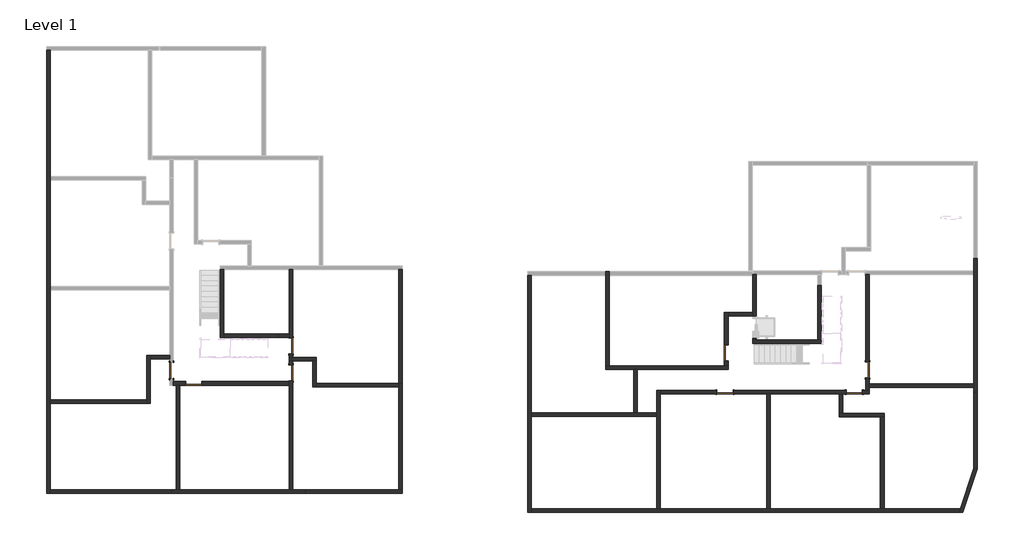
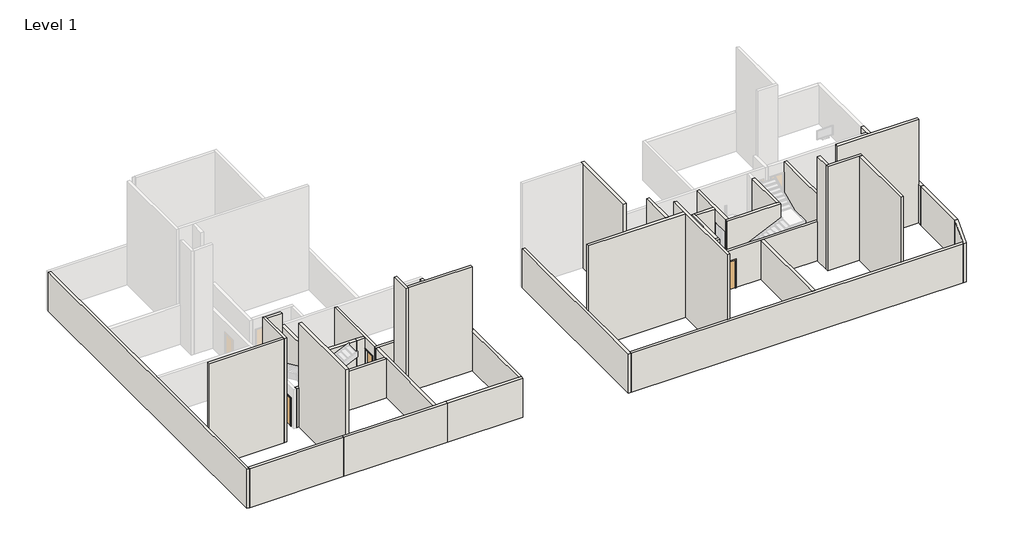
# One storey, part 1 of 2: 41 walls, 8 doors.
"""IFC4 building model written with IfcOpenShell, lengths in millimetres."""

import ifcopenshell
import ifcopenshell.guid

model = None  # the IFC model being written
_history = None  # IfcOwnerHistory: only IFC2X3 demands one
_inside = {}  # id of a spatial element -> (the spatial element, [elements in it])
_under = {}  # id of a project, library or spatial element -> (it, [spatial elements below it])
_declared = {}  # id of a project -> (the project, [libraries it declares])
_typed = {}  # id of a type object -> (the type object, [elements of that type])
_made_of = {}  # id of a material, layer set ... -> (it, [elements and type objects made of it])


def new_model(schema):
    """Start an empty IFC model of exactly this schema.

    Asked for "IFC4X3", IfcOpenShell would pick the latest addendum, in which some entities
    have other attributes; the version numbers below select the first issue.
    IFC2X3 requires an IfcOwnerHistory on every rooted entity: one is made here for all.
    """
    global model, _history
    if schema == "IFC4X3":
        model = ifcopenshell.file(schema_version=(4, 3, 0, 0))
    else:
        model = ifcopenshell.file(schema=schema)
    _inside.clear()
    _under.clear()
    _declared.clear()
    _typed.clear()
    _made_of.clear()
    _history = None
    if model.schema == "IFC2X3":
        org = make("IfcOrganization", Name="unknown")
        user = make(
            "IfcPersonAndOrganization",
            ThePerson=make("IfcPerson", FamilyName="unknown"),
            TheOrganization=org,
        )
        app = make(
            "IfcApplication",
            ApplicationDeveloper=org,
            Version="unknown",
            ApplicationFullName="unknown",
            ApplicationIdentifier="unknown",
        )
        _history = make(
            "IfcOwnerHistory",
            OwningUser=user,
            OwningApplication=app,
            ChangeAction="ADDED",
            CreationDate=0,
        )
    return model


def make(cls, **values):
    """One entity of the class cls with the attributes given. An attribute that is None is left unset."""
    return model.create_entity(
        cls, **{name: value for name, value in values.items() if value is not None}
    )


def rooted(cls, **values):
    """An entity with a GlobalId (a new one), such as an element, a storey or a relation."""
    return make(cls, GlobalId=ifcopenshell.guid.new(), OwnerHistory=_history, **values)


def si_unit(unit_type, name, prefix=None):
    """IfcSIUnit, for example si_unit("LENGTHUNIT", "METRE", prefix="MILLI")."""
    return make("IfcSIUnit", UnitType=unit_type, Prefix=prefix, Name=name)


def assignment(units):
    """IfcUnitAssignment: the units of a project."""
    return None if units is None else make("IfcUnitAssignment", Units=units)


def point(xyz):
    """IfcCartesianPoint."""
    return None if xyz is None else make("IfcCartesianPoint", Coordinates=xyz)


def direction(xyz):
    """IfcDirection."""
    return None if xyz is None else make("IfcDirection", DirectionRatios=xyz)


def frame(location, z_axis=None, x_axis=None):
    """IfcAxis2Placement3D, a coordinate frame: its origin and axes. An axis left out is left unset."""
    return make(
        "IfcAxis2Placement3D",
        Location=point(location),
        Axis=direction(z_axis),
        RefDirection=direction(x_axis),
    )


def origin():
    """The frame at (0, 0, 0) with its axes left unset."""
    return frame((0.0, 0.0, 0.0))


def origin_with_axes():
    """The frame at (0, 0, 0) with the z axis (0, 0, 1) and the x axis (1, 0, 0) written out."""
    return frame((0.0, 0.0, 0.0), z_axis=(0.0, 0.0, 1.0), x_axis=(1.0, 0.0, 0.0))


def place(relative_to, where):
    """IfcLocalPlacement: puts the frame where relative to a parent placement (None: the world)."""
    return make(
        "IfcLocalPlacement", PlacementRelTo=relative_to, RelativePlacement=where
    )


def context(
    kind, dimensions, precision=None, world=None, true_north=None, identifier=None
):
    """IfcGeometricRepresentationContext, for example the 3D "Model" context."""
    return make(
        "IfcGeometricRepresentationContext",
        ContextIdentifier=identifier,
        ContextType=kind,
        CoordinateSpaceDimension=dimensions,
        Precision=precision,
        WorldCoordinateSystem=world,
        TrueNorth=true_north,
    )


def project(units=None, contexts=None):
    """IfcProject with its units and contexts."""
    return rooted(
        "IfcProject",
        Name="project",
        RepresentationContexts=contexts,
        UnitsInContext=assignment(units),
    )


def spatial(cls, under=None, at=None, **own):
    """A site, building, storey or space (cls), placed at a placement, below another one or the project."""
    s = rooted(cls, ObjectPlacement=at, **own)
    if under is not None:
        _under.setdefault(under.id(), (under, []))[1].append(s)
    return s


def polyline(points):
    """IfcPolyline through the points."""
    return make("IfcPolyline", Points=[point(p) for p in points])


def outline(outer, holes=None, kind="AREA"):
    """IfcArbitraryClosedProfileDef: a profile drawn as a closed curve; with holes, ...WithVoids."""
    if holes is None:
        return make("IfcArbitraryClosedProfileDef", ProfileType=kind, OuterCurve=outer)
    return make(
        "IfcArbitraryProfileDefWithVoids",
        ProfileType=kind,
        OuterCurve=outer,
        InnerCurves=holes,
    )


def extrude(swept, where, along, depth):
    """IfcExtrudedAreaSolid: the profile swept, set in the frame where, extruded along a direction by depth."""
    return make(
        "IfcExtrudedAreaSolid",
        SweptArea=swept,
        Position=where,
        ExtrudedDirection=direction(along),
        Depth=depth,
    )


def faces_of(points, faces, orient=None, outer=None):
    """IfcFace entities. A face is a list of loops; a loop is a list of indices into points, from 0.

    orient and outer hold one flag for each loop. By default every Orientation is true, the
    first loop of a face is its IfcFaceOuterBound and the others are IfcFaceBound.
    """
    made = []
    for i, loops in enumerate(faces):
        bounds = []
        for j, loop in enumerate(loops):
            is_outer = j == 0 if outer is None else outer[i][j]
            bounds.append(
                make(
                    "IfcFaceOuterBound" if is_outer else "IfcFaceBound",
                    Bound=make("IfcPolyLoop", Polygon=[points[k] for k in loop]),
                    Orientation=True if orient is None else orient[i][j],
                )
            )
        made.append(make("IfcFace", Bounds=bounds))
    return made


def faceted_brep(points, faces, orient=None, outer=None, voids=None):
    """IfcFacetedBrep: a solid bounded by flat faces; with voids (closed shells), ...WithVoids."""
    shared = [point(p) for p in points]
    hull = make("IfcClosedShell", CfsFaces=faces_of(shared, faces, orient, outer))
    if voids is None:
        return make("IfcFacetedBrep", Outer=hull)
    return make(
        "IfcFacetedBrepWithVoids",
        Outer=hull,
        Voids=[
            make(cls, CfsFaces=faces_of(shared, fs, o, b)) for cls, fs, o, b in voids
        ],
    )


def shape(context_of_items, identifier, shape_type, items):
    """IfcShapeRepresentation: the items that make up one representation, for example the "Body"."""
    return make(
        "IfcShapeRepresentation",
        ContextOfItems=context_of_items,
        RepresentationIdentifier=identifier,
        RepresentationType=shape_type,
        Items=items,
    )


def source(mapping_origin, context_of_items, identifier, shape_type, items):
    """IfcRepresentationMap: a shape defined once, which mapped items show again and again."""
    return make(
        "IfcRepresentationMap",
        MappingOrigin=mapping_origin,
        MappedRepresentation=shape(context_of_items, identifier, shape_type, items),
    )


def transform(
    local_origin,
    x_axis=None,
    y_axis=None,
    z_axis=None,
    scale=None,
    scale2=None,
    scale3=None,
    uniform=True,
):
    """IfcCartesianTransformationOperator3D, or its non-uniform kind. x_axis, y_axis, z_axis: its Axis1, 2, 3."""
    if uniform:
        return make(
            "IfcCartesianTransformationOperator3D",
            Axis1=direction(x_axis),
            Axis2=direction(y_axis),
            LocalOrigin=point(local_origin),
            Scale=scale,
            Axis3=direction(z_axis),
        )
    return make(
        "IfcCartesianTransformationOperator3DnonUniform",
        Axis1=direction(x_axis),
        Axis2=direction(y_axis),
        LocalOrigin=point(local_origin),
        Scale=scale,
        Axis3=direction(z_axis),
        Scale2=scale2,
        Scale3=scale3,
    )


def mapped(mapping_source, mapping_target):
    """IfcMappedItem: shows the shape of a source again, moved by a transform."""
    return make(
        "IfcMappedItem", MappingSource=mapping_source, MappingTarget=mapping_target
    )


def made_of(thing, what):
    """Note that an element or type object is made of a material, layer set ...; save() writes the relation."""
    if what is not None:
        _made_of.setdefault(what.id(), (what, []))[1].append(thing)
    return thing


def element(
    cls,
    number,
    at=None,
    inside=None,
    cuts=None,
    type_object=None,
    material=None,
    context=None,
    identifier="Body",
    shape_type=None,
    held_by="IfcProductDefinitionShape",
    body=None,
    shapes=None,
    **own,
):
    """One element of the class cls, such as IfcWall. Its Tag is "e" and its number.

    at: its placement. inside: the storey or other place that contains it. cuts: it is an
    opening in that element (IfcRelVoidsElement). A single representation is given by context,
    identifier, shape_type and body (its items); several are given by shapes. held_by: the class
    of the entity that holds the representations. save() writes the other relations.
    """
    e = rooted(cls, Tag="e%d" % number, ObjectPlacement=at, **own)
    if body is not None:
        shapes = [shape(context, identifier, shape_type, body)]
    if shapes is not None:
        e.Representation = make(held_by, Representations=shapes)
    if inside is not None:
        _inside.setdefault(inside.id(), (inside, []))[1].append(e)
    if cuts is not None:
        rooted(
            "IfcRelVoidsElement", RelatingBuildingElement=cuts, RelatedOpeningElement=e
        )
    if type_object is not None:
        _typed.setdefault(type_object.id(), (type_object, []))[1].append(e)
    return made_of(e, material)


def aggregate(whole, parts):
    """IfcRelAggregates: a whole, such as a stair, and the parts it consists of."""
    return rooted("IfcRelAggregates", RelatingObject=whole, RelatedObjects=parts)


def save(model, path):
    """Write the relations noted so far, then the file.

    IfcRelAggregates (storeys below a building ...), IfcRelContainedInSpatialStructure (elements
    in a storey), IfcRelDefinesByType, IfcRelAssociatesMaterial and IfcRelDeclares: one each for
    every whole, place, type object, material and project.
    """
    for whole, parts in _under.values():
        aggregate(whole, parts)
    for where, things in _inside.values():
        rooted(
            "IfcRelContainedInSpatialStructure",
            RelatedElements=things,
            RelatingStructure=where,
        )
    for kind, things in _typed.values():
        rooted("IfcRelDefinesByType", RelatedObjects=things, RelatingType=kind)
    for what, things in _made_of.values():
        rooted("IfcRelAssociatesMaterial", RelatedObjects=things, RelatingMaterial=what)
    for by, libraries in _declared.values():
        rooted("IfcRelDeclares", RelatingContext=by, RelatedDefinitions=libraries)
    model.write(path)


def m_single_flush_0915_x_2134mm_727434cd(model_context):
    return source(origin(), model_context, "Body", "SweptSolid", [
        extrude(outline(polyline([(2210.0, -533.5), (0.0, -533.5), (0.0, -457.5), (2134.0, -457.5), (2134.0, 457.5), (0.0, 457.5), (0.0, 533.5), (2210.0, 533.5), (2210.0, -533.5)])), frame((0.0, -125.0, 0.0), z_axis=(0.0, 1.0, 0.0), x_axis=(0.0, 0.0, 1.0)), (0.0, 0.0, 1.0), 25.0),
        extrude(outline(polyline([(2210.0, 533.5), (2210.0, -533.5), (0.0, -533.5), (0.0, -457.5), (2134.0, -457.5), (2134.0, 457.5), (0.0, 457.5), (0.0, 533.5), (2210.0, 533.5)])), frame((0.0, 100.0, 0.0), z_axis=(0.0, 1.0, 0.0), x_axis=(0.0, 0.0, 1.0)), (0.0, 0.0, 1.0), 25.0),
        extrude(outline(polyline([(457.5, -49.0), (457.5, -100.0), (-457.5, -100.0), (-457.5, -49.0), (457.5, -49.0)])), origin_with_axes(), (0.0, 0.0, 1.0), 2134.0),
    ])


def m_single_flush_0915_x_2134mm_6a9e8738(model_context):
    return source(origin(), model_context, "Body", "SweptSolid", [
        extrude(outline(polyline([(2210.0, -533.5), (0.0, -533.5), (0.0, -457.5), (2134.0, -457.5), (2134.0, 457.5), (0.0, 457.5), (0.0, 533.5), (2210.0, 533.5), (2210.0, -533.5)])), frame((0.0, 100.0, 0.0), z_axis=(0.0, 1.0, 0.0), x_axis=(0.0, 0.0, 1.0)), (0.0, 0.0, 1.0), 25.0),
        extrude(outline(polyline([(2210.0, 533.5), (2210.0, -533.5), (0.0, -533.5), (0.0, -457.5), (2134.0, -457.5), (2134.0, 457.5), (0.0, 457.5), (0.0, 533.5), (2210.0, 533.5)])), frame((0.0, -125.0, 0.0), z_axis=(0.0, 1.0, 0.0), x_axis=(0.0, 0.0, 1.0)), (0.0, 0.0, 1.0), 25.0),
        extrude(outline(polyline([(457.5, 49.0), (-457.5, 49.0), (-457.5, 100.0), (457.5, 100.0), (457.5, 49.0)])), origin_with_axes(), (0.0, 0.0, 1.0), 2134.0),
    ])


model = new_model("IFC4")

# Units and contexts
model_context = context("Model", 3, world=origin())
ifc_project = project(units=[si_unit("LENGTHUNIT", "METRE", prefix="MILLI")], contexts=[model_context])

# Site, building, storey
site = spatial("IfcSite", under=ifc_project)
building = spatial("IfcBuilding", under=site)
storey = spatial("IfcBuildingStorey", under=building, Name="Level 1", Elevation=0.0)

# Doors
placement = place(None, origin())
m_single_flush_0915_x_2134mm_shape = m_single_flush_0915_x_2134mm_727434cd(model_context)
element("IfcDoor", 1, ObjectType="M_Single-Flush : 0915 x 2134mm", at=placement, inside=storey, context=model_context, shape_type="MappedRepresentation", body=[
    mapped(m_single_flush_0915_x_2134mm_shape, transform((16070.6041014, -3023.024372, 0.0), x_axis=(0.0, -1.0, 0.0), y_axis=(1.0, 0.0, 0.0), z_axis=(0.0, 0.0, 1.0))),
])
element("IfcDoor", 2, ObjectType="M_Single-Flush : 0915 x 2134mm", at=placement, inside=storey, context=model_context, shape_type="MappedRepresentation", body=[
    mapped(m_single_flush_0915_x_2134mm_shape, transform((16002.336337, -5240.0098119, 0.0), x_axis=(1.0, 0.0, 0.0), y_axis=(0.0, 1.0, 0.0), z_axis=(0.0, 0.0, 1.0))),
])
element("IfcDoor", 3, ObjectType="M_Single-Flush : 0915 x 2134mm", at=placement, inside=storey, context=model_context, shape_type="MappedRepresentation", body=[
    mapped(m_single_flush_0915_x_2134mm_shape, transform((-8530.3449834, -4137.6378151, 0.0), x_axis=(0.0, 1.0, 0.0), y_axis=(-1.0, 0.0, 0.0), z_axis=(0.0, 0.0, 1.0))),
])
m_single_flush_0915_x_2134mm_2_shape = m_single_flush_0915_x_2134mm_6a9e8738(model_context)
element("IfcDoor", 4, ObjectType="M_Single-Flush : 0915 x 2134mm", at=placement, inside=storey, context=model_context, shape_type="MappedRepresentation", body=[
    mapped(m_single_flush_0915_x_2134mm_2_shape, transform((24048.8612349, -3982.5098119, 0.0), x_axis=(0.0, -1.0, 0.0), y_axis=(1.0, 0.0, 0.0), z_axis=(0.0, 0.0, 1.0))),
])
element("IfcDoor", 5, ObjectType="M_Single-Flush : 0915 x 2134mm", at=placement, inside=storey, context=model_context, shape_type="MappedRepresentation", body=[
    mapped(m_single_flush_0915_x_2134mm_2_shape, transform((23308.8612349, -5240.0098119, 0.0), x_axis=(-1.0, 0.0, 0.0), y_axis=(0.0, -1.0, 0.0), z_axis=(0.0, 0.0, 1.0))),
])
element("IfcDoor", 6, ObjectType="M_Single-Flush : 0915 x 2134mm", at=placement, inside=storey, context=model_context, shape_type="MappedRepresentation", body=[
    mapped(m_single_flush_0915_x_2134mm_2_shape, transform((-14032.3304233, -4739.1627129, 0.0), x_axis=(-1.0, 0.0, 0.0), y_axis=(0.0, -1.0, 0.0), z_axis=(0.0, 0.0, 1.0))),
])
element("IfcDoor", 7, ObjectType="M_Single-Flush : 0915 x 2134mm", at=placement, inside=storey, context=model_context, shape_type="MappedRepresentation", body=[
    mapped(m_single_flush_0915_x_2134mm_2_shape, transform((-8530.3449834, -2622.6378151, 0.0), x_axis=(0.0, -1.0, 0.0), y_axis=(1.0, 0.0, 0.0), z_axis=(0.0, 0.0, 1.0))),
])
element("IfcDoor", 8, ObjectType="M_Single-Flush : 0915 x 2134mm", at=placement, inside=storey, context=model_context, shape_type="MappedRepresentation", body=[
    mapped(m_single_flush_0915_x_2134mm_2_shape, transform((-15289.8304233, -3999.1627129, 0.0), x_axis=(0.0, 1.0, 0.0), y_axis=(-1.0, 0.0, 0.0), z_axis=(0.0, 0.0, 1.0))),
])

# Walls
element("IfcWall", 9, ObjectType="Generic - 200mm", at=placement, inside=storey, context=model_context, shape_type="Brep", body=[
    faceted_brep([(30068.8612349, 2319.475628, 0.0), (30068.8612349, 1619.475628, 0.0), (30068.8612349, 1419.475628, 0.0), (30068.8612349, -4760.0098119, 0.0), (30068.8612349, -4960.0098119, 0.0), (30068.8612349, -5240.0098119, 0.0), (30068.8612349, -5240.0098119, 3000.0), (30068.8612349, 1419.475628, 3000.0), (30068.8612349, 1619.475628, 3000.0), (30068.8612349, 2319.475628, 3000.0), (30268.8612349, 2319.475628, 0.0), (30268.8612349, 2319.475628, 3000.0), (30268.8612349, -5240.0098119, 3000.0), (30268.8612349, -5240.0098119, 0.0), (30268.3425199, 2319.475628, 0.0), (30069.3799498, -5240.0098119, 0.0), (30069.3799498, -5240.0098119, 3000.0), (30268.3425199, 2319.475628, 3000.0)], [[[0, 1, 2, 3, 4, 5, 6, 7, 8, 9]], [[10, 11, 12, 13]], [[5, 4, 3, 2, 1, 0, 14, 10, 13, 15]], [[6, 5, 15, 13, 12, 16]], [[9, 8, 7, 6, 16, 12, 11, 17]], [[0, 9, 17, 11, 10, 14]]]),
])
element("IfcWall", 10, ObjectType="Generic - 200mm", at=placement, inside=storey, context=model_context, shape_type="Brep", body=[
    faceted_brep([(30069.3799498, -5240.0098119, 0.0), (30069.3799498, -9543.0251929, 0.0), (30069.3799498, -9543.0251929, 3000.0), (30069.3799498, -5240.0098119, 3000.0), (30269.3799498, -5240.0098119, 0.0), (30269.3799498, -5240.0098119, 3000.0), (30269.3799498, -9575.863443, 3000.0), (30269.3799498, -9575.863443, 0.0), (30268.8612349, -5240.0098119, 0.0), (30268.8612349, -5240.0098119, 3000.0)], [[[0, 1, 2, 3]], [[4, 5, 6, 7]], [[1, 0, 8, 4, 7]], [[3, 2, 6, 5, 9]], [[0, 3, 9, 5, 4, 8]], [[2, 1, 7, 6]]]),
])
element("IfcWall", 11, ObjectType="Generic - 200mm", at=placement, inside=storey, context=model_context, shape_type="Brep", body=[
    faceted_brep([(21449.836337, -2276.2808257, 0.0), (21249.836337, -2276.2808257, 0.0), (17770.6041014, -2276.2808257, 0.0), (17570.6041014, -2276.2808257, 0.0), (17570.6041014, -2276.2808257, 3000.0), (17770.6041014, -2276.2808257, 3000.0), (21249.836337, -2276.2808257, 3000.0), (21449.836337, -2276.2808257, 3000.0), (21449.836337, -2476.2808257, 0.0), (21449.836337, -2476.2808257, 3000.0), (17570.6041014, -2476.2808257, 3000.0), (17570.6041014, -2476.2808257, 0.0)], [[[0, 1, 2, 3, 4, 5, 6, 7]], [[8, 9, 10, 11]], [[3, 2, 1, 0, 8, 11]], [[7, 6, 5, 4, 10, 9]], [[0, 7, 9, 8]], [[4, 3, 11, 10]]]),
])
element("IfcWall", 12, ObjectType="Generic - 200mm", at=placement, inside=storey, context=model_context, shape_type="SweptSolid", body=[
    extrude(outline(polyline([(18559.836337, -5340.0098119), (18559.836337, -11836.6907835), (18359.836337, -11836.6907835), (18359.836337, -5340.0098119), (18559.836337, -5340.0098119)])), origin_with_axes(), (0.0, 0.0, 1.0), 3000.0),
])
element("IfcWall", 13, ObjectType="Generic - 200mm", at=placement, inside=storey, context=model_context, shape_type="Brep", body=[
    faceted_brep([(29295.3124022, -11836.6907835, 0.0), (24988.8612349, -11836.6907835, 0.0), (24788.8612349, -11836.6907835, 0.0), (18559.836337, -11836.6907835, 0.0), (18359.836337, -11836.6907835, 0.0), (12342.1281129, -11836.6907835, 0.0), (12142.1281129, -11836.6907835, 0.0), (5043.716007, -11836.6907835, 0.0), (5043.716007, -11836.6907835, 3000.0), (18359.836337, -11836.6907835, 3000.0), (18559.836337, -11836.6907835, 3000.0), (29295.3124022, -11836.6907835, 3000.0), (29227.8162902, -12036.6907835, 0.0), (29227.8162902, -12036.6907835, 3000.0), (5043.716007, -12036.6907835, 3000.0), (5043.716007, -12036.6907835, 0.0)], [[[0, 1, 2, 3, 4, 5, 6, 7, 8, 9, 10, 11]], [[12, 13, 14, 15]], [[7, 6, 5, 4, 3, 2, 1, 0, 12, 15]], [[11, 10, 9, 8, 14, 13]], [[0, 11, 13, 12]], [[8, 7, 15, 14]]]),
])
element("IfcWall", 14, ObjectType="Generic - 200mm", at=placement, inside=storey, context=model_context, shape_type="Brep", body=[
    faceted_brep([(30069.3799498, -9543.0251929, 0.0), (29295.3124022, -11836.6907835, 0.0), (29227.8162902, -12036.6907835, 0.0), (29227.8162902, -12036.6907835, 3000.0), (29295.3124022, -11836.6907835, 3000.0), (30069.3799498, -9543.0251929, 3000.0), (30269.3799498, -9575.863443, 0.0), (30269.3799498, -9575.863443, 3000.0), (29438.8985612, -12036.6907835, 3000.0), (29438.8985612, -12036.6907835, 0.0)], [[[0, 1, 2, 3, 4, 5]], [[6, 7, 8, 9]], [[2, 1, 0, 6, 9]], [[5, 4, 3, 8, 7]], [[0, 5, 7, 6]], [[3, 2, 9, 8]]]),
])
element("IfcWall", 15, ObjectType="Generic - 200mm", at=placement, inside=storey, context=model_context, shape_type="Brep", body=[
    faceted_brep([(22851.3612349, -5140.0098119, 2134.0), (22851.3612349, -5140.0098119, 0.0), (16459.836337, -5140.0098119, 0.0), (16459.836337, -5140.0098119, 2134.0), (15544.836337, -5140.0098119, 2134.0), (15544.836337, -5140.0098119, 0.0), (12342.1281129, -5140.0098119, 0.0), (12342.1281129, -5140.0098119, 3000.0), (23948.8612349, -5140.0098119, 3000.0), (24148.8612349, -5140.0098119, 3000.0), (24163.3998354, -5140.0098119, 3000.0), (24163.3998354, -5140.0098119, 0.0), (24148.8612349, -5140.0098119, 0.0), (23948.8612349, -5140.0098119, 0.0), (23766.3612349, -5140.0098119, 0.0), (23766.3612349, -5140.0098119, 2134.0), (16459.836337, -5340.0098119, 0.0), (18359.836337, -5340.0098119, 0.0), (18559.836337, -5340.0098119, 0.0), (22468.8612349, -5340.0098119, 0.0), (22668.8612349, -5340.0098119, 0.0), (22851.3612349, -5340.0098119, 0.0), (22851.3612349, -5340.0098119, 2134.0), (23766.3612349, -5340.0098119, 2134.0), (23766.3612349, -5340.0098119, 0.0), (24163.3998354, -5340.0098119, 0.0), (24163.3998354, -5340.0098119, 3000.0), (18559.836337, -5340.0098119, 3000.0), (18359.836337, -5340.0098119, 3000.0), (12342.1281129, -5340.0098119, 3000.0), (12342.1281129, -5340.0098119, 0.0), (15544.836337, -5340.0098119, 0.0), (15544.836337, -5340.0098119, 2134.0), (16459.836337, -5340.0098119, 2134.0)], [[[0, 1, 2, 3, 4, 5, 6, 7, 8, 9, 10, 11, 12, 13, 14, 15]], [[16, 17, 18, 19, 20, 21, 22, 23, 24, 25, 26, 27, 28, 29, 30, 31, 32, 33]], [[2, 1, 21, 20, 19, 18, 17, 16]], [[14, 13, 12, 11, 25, 24]], [[30, 6, 5, 31]], [[10, 9, 8, 7, 29, 28, 27, 26]], [[11, 10, 26, 25]], [[33, 3, 2, 16]], [[4, 32, 31, 5]], [[32, 4, 3, 33]], [[22, 21, 1, 0]], [[23, 22, 0, 15]], [[24, 23, 15, 14]], [[7, 6, 30, 29]]]),
])
element("IfcWall", 16, ObjectType="Generic - 200mm", at=placement, inside=storey, context=model_context, shape_type="Brep", body=[
    faceted_brep([(4843.716007, 1379.9901881, 0.0), (4843.716007, -12036.6907835, 0.0), (4843.716007, -12036.6907835, 3000.0), (4843.716007, 1379.9901881, 3000.0), (5043.716007, 1379.9901881, 0.0), (5043.716007, 1379.9901881, 3000.0), (5043.716007, -11836.6907835, 3000.0), (5043.716007, -12036.6907835, 3000.0), (5043.716007, -12036.6907835, 0.0), (5043.716007, -11836.6907835, 0.0), (5043.716007, -6600.0098119, 0.0), (5043.716007, -6400.0098119, 0.0)], [[[0, 1, 2, 3]], [[4, 5, 6, 7, 8, 9, 10, 11]], [[1, 0, 4, 11, 10, 9, 8]], [[3, 2, 7, 6, 5]], [[2, 1, 8, 7]], [[0, 3, 5, 4]]]),
])
element("IfcWall", 17, ObjectType="Generic - 200mm", at=placement, inside=storey, context=model_context, shape_type="Brep", body=[
    faceted_brep([(24148.8612349, 1419.475628, 3000.0), (24148.8612349, -5140.0098119, 3000.0), (24148.8612349, -5140.0098119, 0.0), (24148.8612349, -4960.0098119, 0.0), (24148.8612349, -4760.0098119, 0.0), (24148.8612349, -4440.0098119, 0.0), (24148.8612349, -4440.0098119, 2134.0), (24148.8612349, -3525.0098119, 2134.0), (24148.8612349, -3525.0098119, 0.0), (24148.8612349, 1419.475628, 0.0), (23948.8612349, -5140.0098119, 3000.0), (23948.8612349, 1419.475628, 3000.0), (23948.8612349, 1419.475628, 0.0), (23948.8612349, -3525.0098119, 0.0), (23948.8612349, -3525.0098119, 2134.0), (23948.8612349, -4440.0098119, 2134.0), (23948.8612349, -4440.0098119, 0.0), (23948.8612349, -5140.0098119, 0.0)], [[[0, 1, 2, 3, 4, 5, 6, 7, 8, 9]], [[10, 11, 12, 13, 14, 15, 16, 17]], [[12, 9, 8, 13]], [[2, 17, 16, 5, 4, 3]], [[1, 0, 11, 10]], [[0, 9, 12, 11]], [[15, 6, 5, 16]], [[7, 14, 13, 8]], [[14, 7, 6, 15]], [[2, 1, 10, 17]]]),
])
element("IfcWall", 18, ObjectType="Generic - 200mm", at=placement, inside=storey, context=model_context, shape_type="SweptSolid", body=[
    extrude(outline(polyline([(21249.836337, -2276.2808257), (21249.836337, 799.475628), (21449.836337, 799.475628), (21449.836337, -2276.2808257), (21249.836337, -2276.2808257)])), origin_with_axes(), (0.0, 0.0, 1.0), 3000.0),
])
element("IfcWall", 19, ObjectType="Generic - 200mm", at=placement, inside=storey, context=model_context, shape_type="Brep", body=[
    faceted_brep([(17570.6041014, -2276.2808257, 3000.0), (17570.6041014, -920.524372, 3000.0), (17570.6041014, -720.524372, 3000.0), (17570.6041014, 1379.475628, 3000.0), (17570.6041014, 1419.475628, 3000.0), (17570.6041014, 1419.475628, 0.0), (17570.6041014, 1379.475628, 0.0), (17570.6041014, -720.524372, 0.0), (17570.6041014, -920.524372, 0.0), (17570.6041014, -926.2808257, 0.0), (17570.6041014, -926.2808257, 2000.0), (17570.6041014, -2181.2876228, 2000.0), (17570.6041014, -2181.2876228, 0.0), (17570.6041014, -2276.2808257, 0.0), (17770.6041014, 1419.475628, 3000.0), (17770.6041014, -2276.2808257, 3000.0), (17770.6041014, -2276.2808257, 0.0), (17770.6041014, -2181.2876228, 0.0), (17770.6041014, -2181.2876228, 2000.0), (17770.6041014, -926.2808257, 2000.0), (17770.6041014, -926.2808257, 0.0), (17770.6041014, 1419.475628, 0.0)], [[[0, 1, 2, 3, 4, 5, 6, 7, 8, 9, 10, 11, 12, 13]], [[14, 15, 16, 17, 18, 19, 20, 21]], [[16, 13, 12, 17]], [[5, 21, 20, 9, 8, 7, 6]], [[4, 3, 2, 1, 0, 15, 14]], [[0, 13, 16, 15]], [[5, 4, 14, 21]], [[11, 18, 17, 12]], [[19, 10, 9, 20]], [[10, 19, 18, 11]]]),
])
element("IfcWall", 20, ObjectType="Generic - 200mm", at=placement, inside=storey, context=model_context, shape_type="Brep", body=[
    faceted_brep([(9268.8612349, -3940.0098119, 0.0), (10830.3209687, -3940.0098119, 0.0), (11030.3209687, -3940.0098119, 0.0), (16170.6041014, -3940.0098119, 0.0), (16170.6041014, -3940.0098119, 3000.0), (9268.8612349, -3940.0098119, 3000.0), (9268.8612349, -3740.0098119, 0.0), (9268.8612349, -3740.0098119, 3000.0), (15970.6041014, -3740.0098119, 3000.0), (16170.6041014, -3740.0098119, 3000.0), (16170.6041014, -3740.0098119, 0.0), (15970.6041014, -3740.0098119, 0.0), (9468.8612349, -3740.0098119, 0.0)], [[[0, 1, 2, 3, 4, 5]], [[6, 7, 8, 9, 10, 11, 12]], [[3, 2, 1, 0, 6, 12, 11, 10]], [[5, 4, 9, 8, 7]], [[4, 3, 10, 9]], [[0, 5, 7, 6]]]),
])
element("IfcWall", 21, ObjectType="Generic - 200mm", at=placement, inside=storey, context=model_context, shape_type="Brep", body=[
    faceted_brep([(16170.6041014, -720.524372, 3000.0), (16170.6041014, -920.524372, 3000.0), (16170.6041014, -3740.0098119, 3000.0), (16170.6041014, -3740.0098119, 0.0), (16170.6041014, -3480.524372, 0.0), (16170.6041014, -3480.524372, 2134.0), (16170.6041014, -2565.524372, 2134.0), (16170.6041014, -2565.524372, 0.0), (16170.6041014, -920.524372, 0.0), (16170.6041014, -720.524372, 0.0), (15970.6041014, -3740.0098119, 3000.0), (15970.6041014, -720.524372, 3000.0), (15970.6041014, -720.524372, 0.0), (15970.6041014, -2565.524372, 0.0), (15970.6041014, -2565.524372, 2134.0), (15970.6041014, -3480.524372, 2134.0), (15970.6041014, -3480.524372, 0.0), (15970.6041014, -3740.0098119, 0.0)], [[[0, 1, 2, 3, 4, 5, 6, 7, 8, 9]], [[10, 11, 12, 13, 14, 15, 16, 17]], [[3, 17, 16, 4]], [[12, 9, 8, 7, 13]], [[2, 1, 0, 11, 10]], [[3, 2, 10, 17]], [[0, 9, 12, 11]], [[15, 5, 4, 16]], [[6, 14, 13, 7]], [[14, 6, 5, 15]]]),
])
element("IfcWall", 22, ObjectType="Generic - 200mm", at=placement, inside=storey, context=model_context, shape_type="SweptSolid", body=[
    extrude(outline(polyline([(17570.6041014, -920.524372), (16170.6041014, -920.524372), (16170.6041014, -720.524372), (17570.6041014, -720.524372), (17570.6041014, -920.524372)])), origin_with_axes(), (0.0, 0.0, 1.0), 3000.0),
])
element("IfcWall", 23, ObjectType="Generic - 200mm", at=placement, inside=storey, context=model_context, shape_type="Brep", body=[
    faceted_brep([(22468.8612349, -6641.2808257, 0.0), (24788.8612349, -6641.2808257, 0.0), (24988.8612349, -6641.2808257, 0.0), (24988.8612349, -6641.2808257, 8000.0), (24788.8612349, -6641.2808257, 8000.0), (22468.8612349, -6641.2808257, 8000.0), (22468.8612349, -6441.2808257, 0.0), (22468.8612349, -6441.2808257, 8000.0), (22668.8612349, -6441.2808257, 8000.0), (24988.8612349, -6441.2808257, 8000.0), (24988.8612349, -6441.2808257, 0.0), (22668.8612349, -6441.2808257, 0.0)], [[[0, 1, 2, 3, 4, 5]], [[6, 7, 8, 9, 10, 11]], [[2, 1, 0, 6, 11, 10]], [[5, 4, 3, 9, 8, 7]], [[3, 2, 10, 9]], [[0, 5, 7, 6]]]),
])
element("IfcWall", 24, ObjectType="Generic - 200mm", at=placement, inside=storey, context=model_context, shape_type="SweptSolid", body=[
    extrude(outline(polyline([(24788.8612349, -11836.6907835), (24788.8612349, -6641.2808257), (24988.8612349, -6641.2808257), (24988.8612349, -11836.6907835), (24788.8612349, -11836.6907835)])), origin_with_axes(), (0.0, 0.0, 1.0), 8000.0),
])
element("IfcWall", 25, ObjectType="Generic - 200mm", at=placement, inside=storey, context=model_context, shape_type="SweptSolid", body=[
    extrude(outline(polyline([(22668.8612349, -5340.0098119), (22668.8612349, -6441.2808257), (22468.8612349, -6441.2808257), (22468.8612349, -5340.0098119), (22668.8612349, -5340.0098119)])), origin_with_axes(), (0.0, 0.0, 1.0), 8000.0),
])
element("IfcWall", 26, ObjectType="Generic - 200mm", at=placement, inside=storey, context=model_context, shape_type="SweptSolid", body=[
    extrude(outline(polyline([(30068.8612349, -4960.0098119), (24148.8612349, -4960.0098119), (24148.8612349, -4760.0098119), (30068.8612349, -4760.0098119), (30068.8612349, -4960.0098119)])), origin_with_axes(), (0.0, 0.0, 1.0), 8000.0),
])
element("IfcWall", 27, ObjectType="Generic - 200mm", at=placement, inside=storey, context=model_context, shape_type="Brep", body=[
    faceted_brep([(9268.8612349, 1579.9901881, 0.0), (9268.8612349, 1379.9901881, 0.0), (9268.8612349, -3740.0098119, 0.0), (9268.8612349, -3740.0098119, 3000.0), (9268.8612349, -3740.0098119, 8000.0), (9268.8612349, 1379.9901881, 8000.0), (9268.8612349, 1579.9901881, 8000.0), (9468.8612349, 1579.9901881, 0.0), (9468.8612349, 1579.9901881, 8000.0), (9468.8612349, -3740.0098119, 8000.0), (9468.8612349, -3740.0098119, 0.0), (9468.8612349, 1379.475628, 0.0), (9468.8612349, 1579.475628, 0.0)], [[[0, 1, 2, 3, 4, 5, 6]], [[7, 8, 9, 10, 11, 12]], [[2, 1, 0, 7, 12, 11, 10]], [[6, 5, 4, 9, 8]], [[4, 3, 2, 10, 9]], [[0, 6, 8, 7]]]),
])
element("IfcWall", 28, ObjectType="Generic - 200mm", at=placement, inside=storey, context=model_context, shape_type="Brep", body=[
    faceted_brep([(12142.1281129, -6400.0098119, 0.0), (11030.3209687, -6400.0098119, 0.0), (10830.3209687, -6400.0098119, 0.0), (5043.716007, -6400.0098119, 0.0), (5043.716007, -6400.0098119, 8000.0), (10830.3209687, -6400.0098119, 8000.0), (11030.3209687, -6400.0098119, 8000.0), (12142.1281129, -6400.0098119, 8000.0), (12142.1281129, -6600.0098119, 0.0), (12142.1281129, -6600.0098119, 8000.0), (5043.716007, -6600.0098119, 8000.0), (5043.716007, -6600.0098119, 0.0)], [[[0, 1, 2, 3, 4, 5, 6, 7]], [[8, 9, 10, 11]], [[3, 2, 1, 0, 8, 11]], [[7, 6, 5, 4, 10, 9]], [[4, 3, 11, 10]], [[0, 7, 9, 8]]]),
])
element("IfcWall", 29, ObjectType="Generic - 200mm", at=placement, inside=storey, context=model_context, shape_type="Brep", body=[
    faceted_brep([(-2430.3449834, -4740.1378151, 0.0), (-2430.3449834, -4940.1378151, 0.0), (-2430.3449834, -10758.643998, 0.0), (-2430.3449834, -10758.643998, 3000.0), (-2430.3449834, -4740.1378151, 3000.0), (-2230.3449834, -4740.1378151, 0.0), (-2230.3449834, -4740.1378151, 3000.0), (-2230.3449834, -10758.643998, 3000.0), (-2230.3449834, -10758.643998, 0.0)], [[[0, 1, 2, 3, 4]], [[5, 6, 7, 8]], [[2, 1, 0, 5, 8]], [[4, 3, 7, 6]], [[3, 2, 8, 7]], [[0, 4, 6, 5]]]),
])
element("IfcWall", 30, ObjectType="Generic - 200mm", at=placement, inside=storey, context=model_context, shape_type="Brep", body=[
    faceted_brep([(-2230.3449834, -10758.643998, 0.0), (-2430.3449834, -10758.643998, 0.0), (-7730.3449834, -10758.643998, 0.0), (-7730.3449834, -10758.643998, 3000.0), (-2430.3449834, -10758.643998, 3000.0), (-2230.3449834, -10758.643998, 3000.0), (-2230.3449834, -10958.643998, 0.0), (-2230.3449834, -10958.643998, 3000.0), (-7730.3449834, -10958.643998, 3000.0), (-7730.3449834, -10958.643998, 0.0), (-7730.3449834, -10759.1627129, 0.0), (-7730.3449834, -10759.1627129, 3000.0)], [[[0, 1, 2, 3, 4, 5]], [[6, 7, 8, 9]], [[2, 1, 0, 6, 9, 10]], [[3, 2, 10, 9, 8, 11]], [[5, 4, 3, 11, 8, 7]], [[0, 5, 7, 6]]]),
])
element("IfcWall", 31, ObjectType="Generic - 200mm", at=placement, inside=storey, context=model_context, shape_type="Brep", body=[
    faceted_brep([(-7730.3449834, -10759.1627129, 0.0), (-8430.3449834, -10759.1627129, 0.0), (-8630.3449834, -10759.1627129, 0.0), (-14809.8304233, -10759.1627129, 0.0), (-15009.8304233, -10759.1627129, 0.0), (-15289.8304233, -10759.1627129, 0.0), (-15289.8304233, -10759.1627129, 3000.0), (-8630.3449834, -10759.1627129, 3000.0), (-8430.3449834, -10759.1627129, 3000.0), (-7730.3449834, -10759.1627129, 3000.0), (-7730.3449834, -10959.1627129, 0.0), (-7730.3449834, -10959.1627129, 3000.0), (-15289.8304233, -10959.1627129, 3000.0), (-15289.8304233, -10959.1627129, 0.0), (-7730.3449834, -10958.643998, 0.0), (-15289.8304233, -10759.6814279, 0.0), (-15289.8304233, -10759.6814279, 3000.0), (-7730.3449834, -10958.643998, 3000.0)], [[[0, 1, 2, 3, 4, 5, 6, 7, 8, 9]], [[10, 11, 12, 13]], [[5, 4, 3, 2, 1, 0, 14, 10, 13, 15]], [[6, 5, 15, 13, 12, 16]], [[9, 8, 7, 6, 16, 12, 11, 17]], [[0, 9, 17, 11, 10, 14]]]),
])
element("IfcWall", 32, ObjectType="Generic - 200mm", at=placement, inside=storey, context=model_context, shape_type="Brep", body=[
    faceted_brep([(-15289.8304233, -10759.6814279, 0.0), (-22146.5113948, -10759.6814279, 0.0), (-22146.5113948, -10759.6814279, 3000.0), (-15289.8304233, -10759.6814279, 3000.0), (-15289.8304233, -10959.6814279, 0.0), (-15289.8304233, -10959.6814279, 3000.0), (-22146.5113948, -10959.6814279, 3000.0), (-22146.5113948, -10959.6814279, 0.0), (-15289.8304233, -10959.1627129, 0.0), (-15289.8304233, -10959.1627129, 3000.0)], [[[0, 1, 2, 3]], [[4, 5, 6, 7]], [[1, 0, 8, 4, 7]], [[3, 2, 6, 5, 9]], [[0, 3, 9, 5, 4, 8]], [[2, 1, 7, 6]]]),
])
element("IfcWall", 33, ObjectType="Generic - 200mm", at=placement, inside=storey, context=model_context, shape_type="Brep", body=[
    faceted_brep([(-12326.101437, -2140.1378151, 0.0), (-12326.101437, -1940.1378151, 0.0), (-12326.101437, 1699.0944206, 0.0), (-12326.101437, 1699.0944206, 3000.0), (-12326.101437, -1940.1378151, 3000.0), (-12326.101437, -2140.1378151, 3000.0), (-12526.101437, -2140.1378151, 0.0), (-12526.101437, -2140.1378151, 3000.0), (-12526.101437, 1699.0944206, 3000.0), (-12526.101437, 1699.0944206, 0.0)], [[[0, 1, 2, 3, 4, 5]], [[6, 7, 8, 9]], [[2, 1, 0, 6, 9]], [[3, 2, 9, 8]], [[5, 4, 3, 8, 7]], [[0, 5, 7, 6]]]),
])
element("IfcWall", 34, ObjectType="Generic - 200mm", at=placement, inside=storey, context=model_context, shape_type="Brep", body=[
    faceted_brep([(-22146.5113948, -10959.6814279, 0.0), (-22146.5113948, -10759.6814279, 0.0), (-22146.5113948, -5879.1627129, 0.0), (-22146.5113948, -5679.1627129, 0.0), (-22146.5113948, 549.8621849, 0.0), (-22146.5113948, 749.8621849, 0.0), (-22146.5113948, 6769.8621849, 0.0), (-22146.5113948, 6969.8621849, 0.0), (-22146.5113948, 14109.8621849, 0.0), (-22146.5113948, 14109.8621849, 3000.0), (-22146.5113948, 6969.8621849, 3000.0), (-22146.5113948, 6769.8621849, 3000.0), (-22146.5113948, 749.8621849, 3000.0), (-22146.5113948, 549.8621849, 3000.0), (-22146.5113948, -10759.6814279, 3000.0), (-22146.5113948, -10959.6814279, 3000.0), (-22346.5113948, -10959.6814279, 0.0), (-22346.5113948, -10959.6814279, 3000.0), (-22346.5113948, 14109.8621849, 3000.0), (-22346.5113948, 14109.8621849, 0.0)], [[[0, 1, 2, 3, 4, 5, 6, 7, 8, 9, 10, 11, 12, 13, 14, 15]], [[16, 17, 18, 19]], [[8, 7, 6, 5, 4, 3, 2, 1, 0, 16, 19]], [[15, 14, 13, 12, 11, 10, 9, 18, 17]], [[9, 8, 19, 18]], [[0, 15, 17, 16]]]),
])
element("IfcWall", 35, ObjectType="Generic - 200mm", at=placement, inside=storey, context=model_context, shape_type="Brep", body=[
    faceted_brep([(-8630.3449834, -4839.1627129, 3000.0), (-15189.8304233, -4839.1627129, 3000.0), (-15189.8304233, -4839.1627129, 0.0), (-15009.8304233, -4839.1627129, 0.0), (-14809.8304233, -4839.1627129, 0.0), (-14489.8304233, -4839.1627129, 0.0), (-14489.8304233, -4839.1627129, 2134.0), (-13574.8304233, -4839.1627129, 2134.0), (-13574.8304233, -4839.1627129, 0.0), (-8630.3449834, -4839.1627129, 0.0), (-15189.8304233, -4639.1627129, 3000.0), (-8630.3449834, -4639.1627129, 3000.0), (-8630.3449834, -4639.1627129, 0.0), (-13574.8304233, -4639.1627129, 0.0), (-13574.8304233, -4639.1627129, 2134.0), (-14489.8304233, -4639.1627129, 2134.0), (-14489.8304233, -4639.1627129, 0.0), (-15189.8304233, -4639.1627129, 0.0)], [[[0, 1, 2, 3, 4, 5, 6, 7, 8, 9]], [[10, 11, 12, 13, 14, 15, 16, 17]], [[12, 9, 8, 13]], [[2, 17, 16, 5, 4, 3]], [[1, 0, 11, 10]], [[0, 9, 12, 11]], [[15, 6, 5, 16]], [[7, 14, 13, 8]], [[14, 7, 6, 15]], [[2, 1, 10, 17]]]),
])
element("IfcWall", 36, ObjectType="Generic - 200mm", at=placement, inside=storey, context=model_context, shape_type="SweptSolid", body=[
    extrude(outline(polyline([(-12326.101437, -1940.1378151), (-9250.3449834, -1940.1378151), (-9250.3449834, -2140.1378151), (-12326.101437, -2140.1378151), (-12326.101437, -1940.1378151)])), origin_with_axes(), (0.0, 0.0, 1.0), 3000.0),
])
element("IfcWall", 37, ObjectType="Generic - 200mm", at=placement, inside=storey, context=model_context, shape_type="SweptSolid", body=[
    extrude(outline(polyline([(-8630.3449834, -2140.1378151), (-9250.3449834, -2140.1378151), (-9250.3449834, -1940.1378151), (-8630.3449834, -1940.1378151), (-8630.3449834, -2140.1378151)])), origin_with_axes(), (0.0, 0.0, 1.0), 3000.0),
])
element("IfcWall", 38, ObjectType="Generic - 200mm", at=placement, inside=storey, context=model_context, shape_type="SweptSolid", body=[
    extrude(outline(polyline([(-2430.3449834, -4740.1378151), (-2430.3449834, 1700.8372871), (-2230.3449834, 1700.8372871), (-2230.3449834, -4740.1378151), (-2430.3449834, -4740.1378151)])), origin_with_axes(), (0.0, 0.0, 1.0), 3000.0),
])
element("IfcWall", 39, ObjectType="Generic - 200mm", at=placement, inside=storey, context=model_context, shape_type="Brep", body=[
    faceted_brep([(-8630.3449834, -3480.1378151, 0.0), (-8430.3449834, -3480.1378151, 0.0), (-7295.3449834, -3480.1378151, 0.0), (-7095.3449834, -3480.1378151, 0.0), (-7095.3449834, -3480.1378151, 3000.0), (-8430.3449834, -3480.1378151, 3000.0), (-8630.3449834, -3480.1378151, 3000.0), (-8630.3449834, -3280.1378151, 0.0), (-8630.3449834, -3280.1378151, 3000.0), (-8430.3449834, -3280.1378151, 3000.0), (-7095.3449834, -3280.1378151, 3000.0), (-7095.3449834, -3280.1378151, 0.0), (-8430.3449834, -3280.1378151, 0.0)], [[[0, 1, 2, 3, 4, 5, 6]], [[7, 8, 9, 10, 11, 12]], [[3, 2, 1, 0, 7, 12, 11]], [[6, 5, 4, 10, 9, 8]], [[0, 6, 8, 7]], [[4, 3, 11, 10]]]),
])
element("IfcWall", 40, ObjectType="Generic - 200mm", at=placement, inside=storey, context=model_context, shape_type="Brep", body=[
    faceted_brep([(-8630.3449834, -10759.1627129, 3000.0), (-8630.3449834, -4839.1627129, 3000.0), (-8630.3449834, -4639.1627129, 3000.0), (-8630.3449834, -3480.1378151, 3000.0), (-8630.3449834, -3480.1378151, 0.0), (-8630.3449834, -3680.1378151, 0.0), (-8630.3449834, -3680.1378151, 2134.0), (-8630.3449834, -4595.1378151, 2134.0), (-8630.3449834, -4595.1378151, 0.0), (-8630.3449834, -4639.1627129, 0.0), (-8630.3449834, -4839.1627129, 0.0), (-8630.3449834, -10759.1627129, 0.0), (-8430.3449834, -3480.1378151, 3000.0), (-8430.3449834, -10759.1627129, 3000.0), (-8430.3449834, -10759.1627129, 0.0), (-8430.3449834, -4595.1378151, 0.0), (-8430.3449834, -4595.1378151, 2134.0), (-8430.3449834, -3680.1378151, 2134.0), (-8430.3449834, -3680.1378151, 0.0), (-8430.3449834, -3480.1378151, 0.0)], [[[0, 1, 2, 3, 4, 5, 6, 7, 8, 9, 10, 11]], [[12, 13, 14, 15, 16, 17, 18, 19]], [[14, 11, 10, 9, 8, 15]], [[4, 19, 18, 5]], [[3, 2, 1, 0, 13, 12]], [[0, 11, 14, 13]], [[4, 3, 12, 19]], [[17, 6, 5, 18]], [[7, 16, 15, 8]], [[16, 7, 6, 17]]]),
])
element("IfcWall", 41, ObjectType="Generic - 200mm", at=placement, inside=storey, context=model_context, shape_type="Brep", body=[
    faceted_brep([(-8430.3449834, 1700.8372871, 3000.0), (-8430.3449834, -3280.1378151, 3000.0), (-8430.3449834, -3280.1378151, 0.0), (-8430.3449834, -3080.1378151, 0.0), (-8430.3449834, -3080.1378151, 2134.0), (-8430.3449834, -2165.1378151, 2134.0), (-8430.3449834, -2165.1378151, 0.0), (-8430.3449834, 1700.8372871, 0.0), (-8630.3449834, -3280.1378151, 3000.0), (-8630.3449834, -2140.1378151, 3000.0), (-8630.3449834, -1940.1378151, 3000.0), (-8630.3449834, 1700.8372871, 3000.0), (-8630.3449834, 1700.8372871, 0.0), (-8630.3449834, -1940.1378151, 0.0), (-8630.3449834, -2140.1378151, 0.0), (-8630.3449834, -2165.1378151, 0.0), (-8630.3449834, -2165.1378151, 2134.0), (-8630.3449834, -3080.1378151, 2134.0), (-8630.3449834, -3080.1378151, 0.0), (-8630.3449834, -3280.1378151, 0.0)], [[[0, 1, 2, 3, 4, 5, 6, 7]], [[8, 9, 10, 11, 12, 13, 14, 15, 16, 17, 18, 19]], [[2, 19, 18, 3]], [[12, 7, 6, 15, 14, 13]], [[1, 0, 11, 10, 9, 8]], [[2, 1, 8, 19]], [[17, 4, 3, 18]], [[5, 16, 15, 6]], [[16, 5, 4, 17]], [[0, 7, 12, 11]]]),
])
element("IfcWall", 42, ObjectType="Generic - 200mm", at=placement, inside=storey, context=model_context, shape_type="Brep", body=[
    faceted_brep([(-7295.3449834, -3480.1378151, 0.0), (-7295.3449834, -4940.1378151, 0.0), (-7295.3449834, -4940.1378151, 8000.0), (-7295.3449834, -3480.1378151, 8000.0), (-7095.3449834, -3480.1378151, 0.0), (-7095.3449834, -3480.1378151, 3000.0), (-7095.3449834, -3480.1378151, 8000.0), (-7095.3449834, -4740.1378151, 8000.0), (-7095.3449834, -4940.1378151, 8000.0), (-7095.3449834, -4940.1378151, 0.0), (-7095.3449834, -4740.1378151, 0.0)], [[[0, 1, 2, 3]], [[4, 5, 6, 7, 8, 9, 10]], [[1, 0, 4, 10, 9]], [[3, 2, 8, 7, 6]], [[2, 1, 9, 8]], [[0, 3, 6, 5, 4]]]),
])
element("IfcWall", 43, ObjectType="Generic - 200mm", at=placement, inside=storey, context=model_context, shape_type="Brep", body=[
    faceted_brep([(-7095.3449834, -4940.1378151, 0.0), (-2430.3449834, -4940.1378151, 0.0), (-2430.3449834, -4940.1378151, 8000.0), (-7095.3449834, -4940.1378151, 8000.0), (-7095.3449834, -4740.1378151, 0.0), (-7095.3449834, -4740.1378151, 8000.0), (-2430.3449834, -4740.1378151, 8000.0), (-2430.3449834, -4740.1378151, 3000.0), (-2430.3449834, -4740.1378151, 0.0)], [[[0, 1, 2, 3]], [[4, 5, 6, 7, 8]], [[1, 0, 4, 8]], [[3, 2, 6, 5]], [[0, 3, 5, 4]], [[2, 1, 8, 7, 6]]]),
])
element("IfcWall", 44, ObjectType="Generic - 200mm", at=placement, inside=storey, context=model_context, shape_type="Brep", body=[
    faceted_brep([(-16691.101437, -3159.1627129, 0.0), (-16691.101437, -5679.1627129, 0.0), (-16691.101437, -5879.1627129, 0.0), (-16691.101437, -5879.1627129, 8000.0), (-16691.101437, -5679.1627129, 8000.0), (-16691.101437, -3159.1627129, 8000.0), (-16491.101437, -3159.1627129, 0.0), (-16491.101437, -3159.1627129, 8000.0), (-16491.101437, -3359.1627129, 8000.0), (-16491.101437, -5879.1627129, 8000.0), (-16491.101437, -5879.1627129, 0.0), (-16491.101437, -3359.1627129, 0.0)], [[[0, 1, 2, 3, 4, 5]], [[6, 7, 8, 9, 10, 11]], [[2, 1, 0, 6, 11, 10]], [[5, 4, 3, 9, 8, 7]], [[3, 2, 10, 9]], [[0, 5, 7, 6]]]),
])
element("IfcWall", 45, ObjectType="Generic - 200mm", at=placement, inside=storey, context=model_context, shape_type="SweptSolid", body=[
    extrude(outline(polyline([(-22146.5113948, -5679.1627129), (-16691.101437, -5679.1627129), (-16691.101437, -5879.1627129), (-22146.5113948, -5879.1627129), (-22146.5113948, -5679.1627129)])), origin_with_axes(), (0.0, 0.0, 1.0), 8000.0),
])
element("IfcWall", 46, ObjectType="Generic - 200mm", at=placement, inside=storey, context=model_context, shape_type="SweptSolid", body=[
    extrude(outline(polyline([(-15389.8304233, -3359.1627129), (-16491.101437, -3359.1627129), (-16491.101437, -3159.1627129), (-15389.8304233, -3159.1627129), (-15389.8304233, -3359.1627129)])), origin_with_axes(), (0.0, 0.0, 1.0), 8000.0),
])
element("IfcWall", 47, ObjectType="Generic - 200mm", at=placement, inside=storey, context=model_context, shape_type="SweptSolid", body=[
    extrude(outline(polyline([(-15009.8304233, -10759.1627129), (-15009.8304233, -4839.1627129), (-14809.8304233, -4839.1627129), (-14809.8304233, -10759.1627129), (-15009.8304233, -10759.1627129)])), origin_with_axes(), (0.0, 0.0, 1.0), 8000.0),
])
element("IfcWall", 48, ObjectType="Generic - 200mm", at=placement, inside=storey, context=model_context, shape_type="Brep", body=[
    faceted_brep([(12142.1281129, -5136.6907835, 0.0), (12142.1281129, -6400.0098119, 0.0), (12142.1281129, -6600.0098119, 0.0), (12142.1281129, -11836.6907835, 0.0), (12142.1281129, -11836.6907835, 8000.0), (12142.1281129, -6600.0098119, 8000.0), (12142.1281129, -6400.0098119, 8000.0), (12142.1281129, -5136.6907835, 8000.0), (12342.1281129, -5136.6907835, 0.0), (12342.1281129, -5136.6907835, 8000.0), (12342.1281129, -11836.6907835, 8000.0), (12342.1281129, -11836.6907835, 0.0), (12342.1281129, -5340.0098119, 0.0), (12342.1281129, -5140.0098119, 0.0)], [[[0, 1, 2, 3, 4, 5, 6, 7]], [[8, 9, 10, 11, 12, 13]], [[3, 2, 1, 0, 8, 13, 12, 11]], [[7, 6, 5, 4, 10, 9]], [[0, 7, 9, 8]], [[4, 3, 11, 10]]]),
])
element("IfcWall", 49, ObjectType="Generic - 200mm", at=placement, inside=storey, context=model_context, shape_type="SweptSolid", body=[
    extrude(outline(polyline([(10830.3209687, -6400.0098119), (10830.3209687, -3940.0098119), (11030.3209687, -3940.0098119), (11030.3209687, -6400.0098119), (10830.3209687, -6400.0098119)])), origin_with_axes(), (0.0, 0.0, 1.0), 8000.0),
])

save(model, "model.ifc")

# Revit data of these elements
# Project information
#   Project Issue Date = "Issue Date"
#   Project Status = "Project Status"
#   Client Name = "Owner"
#   Project Address = "Enter address here"
#   Project Name = "Project Name"
#   Project Number = "0001"
# Type "M_Single-Flush : 0915 x 2134mm"
#   Type Mark = "20"
#   Construction Type Id = "MDOOR"
#   Analytic Construction = "Metal"
#   Thickness = 5.1 cm
#   Thermal Resistance (R) = 0.270117 (m²·K)/W
#   Heat Transfer Coefficient (U) = 3.7021 W/(m²·K)
#   Height = 213.4 cm
#   Trim Projection Ext = 2.5 cm
#   Trim Projection Int = 2.5 cm
#   Trim Width = 7.6 cm
#   Width = 91.5 cm
#   Define Thermal Properties by = 1
#   Define Thermal Properties by = 1
#   Door Material = Door - Panel
#   Frame Material = Door - Frame
#   Visual Light Transmittance = 0
#   Solar Heat Gain Coefficient = 0
#   Function = (empty or 0)
#   Wall Closure = (empty or 0)
# Type "Generic - 200mm"
#   Layers, outside or top first: 20 cm no material (function 1)
# Elements 1, 2, 3, 4, 5, 6, 7, 8 (IfcDoor, "M_Single-Flush : 0915 x 2134mm")
#   Phase Created = New Construction
#   Materials on its faces: "Door - Frame", "Door - Panel"
# Elements 9, 10, 11, 12, 13, 14, 15, 16, 17, 18, 19, 20, 21, 22, 29, 30, 31, 32, 33, 34, 35, 36, 37, 38, 39, 40, 41 (IfcWall, "Generic - 200mm")
#   Top Offset = 0 cm
#   Base Offset = 0 cm
#   wall height = 300 cm
#   Phase Created = New Construction
#   Base Constraint = Level 1
#   Top Constraint = Level 2
#   Materials on its faces: "Default Wall"
# Elements 23, 24, 25, 26, 27, 28, 42, 43, 44, 45, 46, 47, 48, 49 (IfcWall, "Generic - 200mm")
#   Top Offset = 0 cm
#   Base Offset = 0 cm
#   Unconnected Height = 800 cm
#   wall height = 800 cm
#   Phase Created = New Construction
#   Base Constraint = Level 1
#   Materials on its faces: "Default Wall"
# Materials
#   "Door - Panel": class "Wood", colour RGB 210 159 95, transparency 0, Cost = 0
#   "Door - Frame": class "Miscellaneous", colour RGB 118 70 51, transparency 0, Cost = 0
#   "Default Wall": class "Miscellaneous", colour RGB 128 128 128, transparency 0, Cost = 0
# Room, not placed, phase "New Construction", upper offset 0 cm, lower offset 0 cm
#   Number = "11"
#   Name = "Room"
# Room, not placed, phase "New Construction", upper offset 0 cm, lower offset 0 cm
#   Number = "12"
#   Name = "Room"
# Room, not placed, phase "New Construction", upper offset 0 cm, lower offset 0 cm
#   Number = "13"
#   Name = "Room"
# Room, not placed, phase "New Construction", upper offset 0 cm, lower offset 0 cm
#   Number = "14"
#   Name = "Room"
# Room, not placed, phase "New Construction", upper offset 0 cm, lower offset 0 cm
#   Number = "15"
#   Name = "Room"
# Room, not placed, phase "New Construction", upper offset 0 cm, lower offset 0 cm
#   Number = "16"
#   Name = "Room"
# Room, not placed, phase "New Construction", upper offset 0 cm, lower offset 0 cm
#   Number = "30"
#   Name = "Room"
# Room, not placed, phase "New Construction", upper offset 0 cm, lower offset 0 cm
#   Number = "31"
#   Name = "Room"
# Area at (10805.296, 137.532) mm, upper offset 243.84 cm, lower offset 0 cm
#   Number = "4"
#   Name = "Dere Parsel Toplam Alan"
# Room, not placed, phase "New Construction", upper offset 0 cm, lower offset 0 cm
#   Number = "106"
#   Name = "Room"
# Room, not placed, phase "New Construction", upper offset 0 cm, lower offset 0 cm
#   Number = "107"
#   Name = "Room"
# Room, not placed, phase "New Construction", upper offset 0 cm, lower offset 0 cm
#   Number = "109"
#   Name = "Room"
# Room, not placed, phase "New Construction", upper offset 0 cm, lower offset 0 cm
#   Number = "110"
#   Name = "7"
# Room, not placed, phase "New Construction", upper offset 0 cm, lower offset 0 cm
#   Number = "111"
#   Name = "8"
# Room, not placed, phase "New Construction", upper offset 0 cm, lower offset 0 cm
#   Number = "112"
#   Name = "9"
# Room, not placed, phase "New Construction", upper offset 0 cm, lower offset 0 cm
#   Number = "113"
#   Name = "1"
# Room, not placed, phase "New Construction", upper offset 0 cm, lower offset 0 cm
#   Number = "114"
#   Name = "5"
# Room at (-13122.389, -6232.807) mm, phase "New Construction", upper level "Level 1", upper offset 243.84 cm, lower offset 0 cm
#   Number = "115"
#   Name = "2"
# Room, not placed, phase "New Construction", upper offset 0 cm, lower offset 0 cm
#   Number = "116"
#   Name = "4"
# Room at (-18030.351, -8408.051) mm, phase "New Construction", upper level "Level 1", upper offset 243.84 cm, lower offset 0 cm
#   Number = "117"
#   Name = "3"
# Room, not placed, phase "New Construction", upper offset 0 cm, lower offset 0 cm
#   Number = "118"
#   Name = "6"
# Room, not placed, phase "New Construction", upper offset 0 cm, lower offset 0 cm
#   Number = "17"
#   Name = "Room"
# Room, not placed, phase "New Construction", upper offset 0 cm, lower offset 0 cm
#   Number = "119"
#   Name = "Room"
# Room, not placed, phase "New Construction", upper offset 0 cm, lower offset 0 cm
#   Number = "120"
#   Name = "Room"
# Room, not placed, phase "New Construction", upper offset 0 cm, lower offset 0 cm
#   Number = "77"
#   Name = "7"
# Room at (12006.755, -2663.043) mm, phase "New Construction", upper level "Level 1", upper offset 243.84 cm, lower offset 0 cm
#   Number = "78"
#   Name = "8"
# Room at (20215.408, 4344.32) mm, phase "New Construction", upper level "Level 1", upper offset 243.84 cm, lower offset 0 cm
#   Number = "79"
#   Name = "9"
# Room at (24094.982, 2386.264) mm, phase "New Construction", upper level "Level 1", upper offset 243.84 cm, lower offset 0 cm
#   Number = "80"
#   Name = "1"
# Room, not placed, phase "New Construction", upper offset 0 cm, lower offset 0 cm
#   Number = "81"
#   Name = "Room"
# Room, not placed, phase "New Construction", upper offset 0 cm, lower offset 0 cm
#   Number = "82"
#   Name = "Room"
# Room, not placed, phase "New Construction", upper offset 0 cm, lower offset 0 cm
#   Number = "83"
#   Name = "Room"
# Room, not placed, phase "New Construction", upper offset 0 cm, lower offset 0 cm
#   Number = "84"
#   Name = "5"
# Room, not placed, phase "New Construction", upper offset 0 cm, lower offset 0 cm
#   Number = "85"
#   Name = "Room"
# Room, not placed, phase "New Construction", upper offset 0 cm, lower offset 0 cm
#   Number = "18"
#   Name = "Room"
# Room, not placed, phase "New Construction", upper offset 0 cm, lower offset 0 cm
#   Number = "86"
#   Name = "Room"
# Room at (16096.482, -8926.883) mm, phase "New Construction", upper level "Level 1", upper offset 243.84 cm, lower offset 0 cm
#   Number = "121"
#   Name = "Room"
# Room at (9090.309, -9568.804) mm, phase "New Construction", upper level "Level 1", upper offset 243.84 cm, lower offset 0 cm
#   Number = "122"
#   Name = "Room"
# Room at (20160.22, -678.403) mm, phase "New Construction", upper level "Level 1", upper offset 243.84 cm, lower offset 0 cm
#   Number = ""
#   Name = "ASANSÖR"
# Room at (18614.214, -3908.781) mm, phase "New Construction", upper level "Level 1", upper offset 243.84 cm, lower offset 0 cm
#   Number = "49"
#   Name = "Room"
# Room, not placed, phase "New Construction", upper offset 0 cm, lower offset 0 cm
#   Number = "50"
#   Name = "Room"
# Room, not placed, phase "New Construction", upper offset 0 cm, lower offset 0 cm
#   Number = "51"
#   Name = "Room"
# Room, not placed, phase "New Construction", upper offset 0 cm, lower offset 0 cm
#   Number = "52"
#   Name = "Room"
# Room, not placed, phase "New Construction", upper offset 0 cm, lower offset 0 cm
#   Number = "53"
#   Name = "Room"
# Room, not placed, phase "New Construction", upper offset 0 cm, lower offset 0 cm
#   Number = "54"
#   Name = "Room"
# Room, not placed, phase "New Construction", upper offset 0 cm, lower offset 0 cm
#   Number = "55"
#   Name = "Room"
# Room, not placed, phase "New Construction", upper offset 0 cm, lower offset 0 cm
#   Number = "56"
#   Name = "Room"
# Room, not placed, phase "New Construction", upper offset 0 cm, lower offset 0 cm
#   Number = ""
#   Name = "Çamaşır- Kombi"
# Room, not placed, phase "New Construction", upper offset 0 cm, lower offset 0 cm
#   Number = "32"
#   Name = "Room"
# Room, not placed, phase "New Construction", upper offset 0 cm, lower offset 0 cm
#   Number = "33"
#   Name = "Room"
# Room at (7273.818, -4665.691) mm, phase "New Construction", upper level "Level 1", upper offset 243.84 cm, lower offset 0 cm
#   Number = "123"
#   Name = "Room"
# Room at (25542.506, -3072.569) mm, phase "New Construction", upper level "Level 1", upper offset 243.84 cm, lower offset 0 cm
#   Number = "87"
#   Name = "2"
# Room at (21925.305, -9013.945) mm, phase "New Construction", upper level "Level 1", upper offset 243.84 cm, lower offset 0 cm
#   Number = "88"
#   Name = "4"
# Room, not placed, phase "New Construction", upper offset 0 cm, lower offset 0 cm
#   Number = "57"
#   Name = "Room"
# Room, not placed, phase "New Construction", upper offset 0 cm, lower offset 0 cm
#   Number = ""
#   Name = "Room"
# Room, not placed, phase "New Construction", upper offset 0 cm, lower offset 0 cm
#   Number = "59"
#   Name = "Room"
# Room, not placed, phase "New Construction", upper offset 0 cm, lower offset 0 cm
#   Number = "60"
#   Name = "Room"
# Room, not placed, phase "New Construction", upper offset 0 cm, lower offset 0 cm
#   Number = "61"
#   Name = "Room"
# Room, not placed, phase "New Construction", upper offset 0 cm, lower offset 0 cm
#   Number = "62"
#   Name = "Room"
# Room, not placed, phase "New Construction", upper offset 0 cm, lower offset 0 cm
#   Number = "63"
#   Name = "Room"
# Area, not placed, upper offset 0 cm, lower offset 0 cm
#   Number = "5"
#   Name = "Dere Parsel Toplam Alan"
# Room, not placed, phase "New Construction", upper offset 0 cm, lower offset 0 cm
#   Number = "67"
#   Name = "Room"
# Room, not placed, phase "New Construction", upper offset 0 cm, lower offset 0 cm
#   Number = "68"
#   Name = "Room"
# Room at (27717.749, -7980.531) mm, phase "New Construction", upper level "Level 1", upper offset 243.84 cm, lower offset 0 cm
#   Number = "90"
#   Name = "3"
# Area, not placed, upper offset 0 cm, lower offset 0 cm
#   Number = "6"
#   Name = "Area"
# Room, not placed, phase "New Construction", upper offset 0 cm, lower offset 0 cm
#   Number = "93"
#   Name = "6"
# Room, not placed, phase "New Construction", upper offset 0 cm, lower offset 0 cm
#   Number = "5"
#   Name = "Room"
# Room, not placed, phase "New Construction", upper offset 0 cm, lower offset 0 cm
#   Number = "6"
#   Name = "Room"
# Room at (-9476.825, 5160.6) mm, phase "New Construction", upper level "Level 1", upper offset 243.84 cm, lower offset 0 cm
#   Number = "124"
#   Name = "Room"
# Room, not placed, phase "New Construction", upper offset 0 cm, lower offset 0 cm
#   Number = "34"
#   Name = "Room"
# Room, not placed, phase "New Construction", upper offset 0 cm, lower offset 0 cm
#   Number = "35"
#   Name = "Room"
# Room, not placed, phase "New Construction", upper offset 0 cm, lower offset 0 cm
#   Number = "9"
#   Name = "Room"
# Room, not placed, phase "New Construction", upper offset 0 cm, lower offset 0 cm
#   Number = "10"
#   Name = "Room"
# Room, not placed, phase "New Construction", upper offset 0 cm, lower offset 0 cm
#   Number = "125"
#   Name = "Room"
# Room, not placed, phase "New Construction", upper offset 0 cm, lower offset 0 cm
#   Number = "126"
#   Name = "Room"
# Room, not placed, phase "New Construction", upper offset 0 cm, lower offset 0 cm
#   Number = "127"
